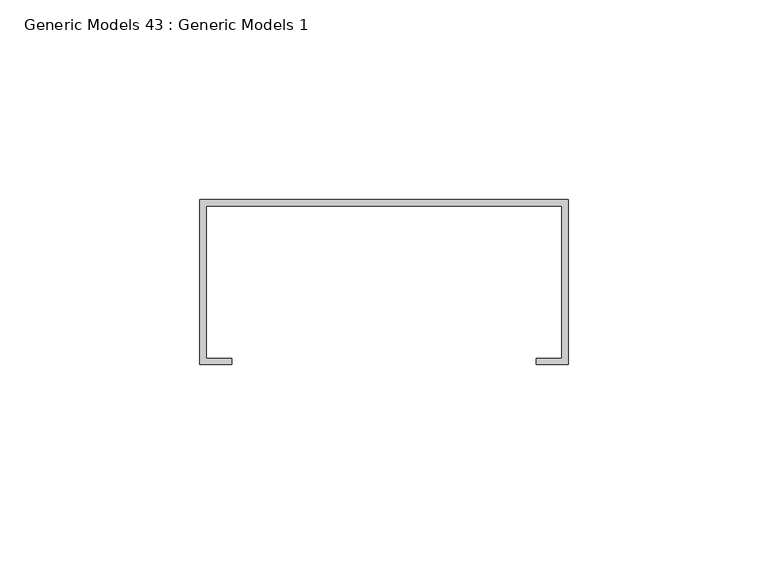
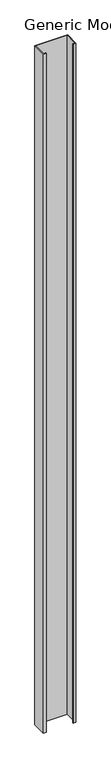
"""IFC4 building model written with IfcOpenShell, lengths in millimetres: proxy geometry, Generic Models 43 : Generic Models 1."""

from ifc_helpers import new_model, si_unit, frame, origin, place, context, project, spatial, polyline, outline, extrude, source, transform, mapped, element, save


def generic_models_43_generic_models_1_113e5eee(model_context):
    return source(origin(), model_context, "Body", "SweptSolid", [
        extrude(outline(polyline([(51003.2, 630.2375), (51003.2, 588.9625), (50995.2625, 588.9625), (50995.2625, 590.55), (51001.6125, 590.55), (51001.6125, 628.65), (50912.7125, 628.65), (50912.7125, 590.55), (50919.0625, 590.55), (50919.0625, 588.9625), (50911.125, 588.9625), (50911.125, 630.2375), (51003.2, 630.2375)])), frame((0.0, 0.0, 1.5875), z_axis=(0.0, 0.0, 1.0), x_axis=(1.0, 0.0, 0.0)), (0.0, 0.0, 1.0), 2025.65),
    ])


if __name__ == "__main__":
    model = new_model("IFC4")
    model_context = context("Model", 3, world=origin())
    ifc_project = project(units=[si_unit("LENGTHUNIT", "METRE", prefix="MILLI")], contexts=[model_context])
    site = spatial("IfcSite", under=ifc_project)
    building = spatial("IfcBuilding", under=site)
    placement = place(None, origin())
    generic_models_43_generic_models_1_shape = generic_models_43_generic_models_1_113e5eee(model_context)
    element("IfcBuildingElementProxy", 1, Name="Generic Models 43 : Generic Models 1", ObjectType="Generic Models 43 : Generic Models 1", at=placement, inside=building, context=model_context, shape_type="MappedRepresentation", body=[
        mapped(generic_models_43_generic_models_1_shape, transform((0.0, 0.0, 0.0), x_axis=(1.0, 0.0, 0.0), y_axis=(0.0, 1.0, 0.0), z_axis=(0.0, 0.0, 1.0))),
    ])
    save(model, "model.ifc")

# Revit data of these elements
# Element 1 (IfcBuildingElementProxy, "Generic Models 43 : Generic Models 1")
#   Materials on its faces: "METAL STUDS (MATCH EXISTING SIZE/GAUGE/SPACING)"
# Materials
#   "METAL STUDS (MATCH EXISTING SIZE/GAUGE/SPACING)": class "Unassigned", colour RGB 210 209 208, transparency 0, Keynote = "M05121300.02", Cost = 0
